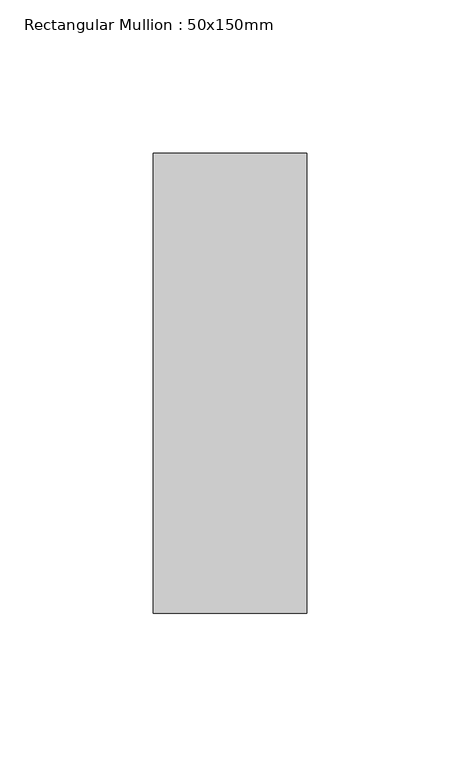
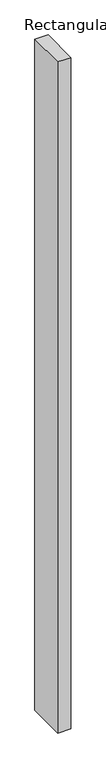
"""IFC4 building model written with IfcOpenShell, lengths in millimetres: member geometry, Rectangular Mullion : 50x150mm."""

from ifc_helpers import new_model, si_unit, frame, origin, place, context, project, spatial, polyline, outline, extrude, source, transform, mapped, element, save


def rectangular_mullion_50x150mm_929c4ac2(model_context):
    return source(origin(), model_context, "Body", "SweptSolid", [
        extrude(outline(polyline([(0.0, 75.0), (0.0, -75.0), (-50.0, -75.0), (-50.0, 75.0), (0.0, 75.0)])), frame((0.0, 0.0, -2700.0), z_axis=(0.0, 0.0, 1.0), x_axis=(1.0, 0.0, 0.0)), (0.0, 0.0, 1.0), 2700.0),
    ])


if __name__ == "__main__":
    model = new_model("IFC4")
    model_context = context("Model", 3, world=origin())
    ifc_project = project(units=[si_unit("LENGTHUNIT", "METRE", prefix="MILLI")], contexts=[model_context])
    site = spatial("IfcSite", under=ifc_project)
    building = spatial("IfcBuilding", under=site)
    placement = place(None, origin())
    rectangular_mullion_50x150mm_shape = rectangular_mullion_50x150mm_929c4ac2(model_context)
    element("IfcMember", 1, ObjectType="Rectangular Mullion : 50x150mm", at=placement, inside=building, context=model_context, shape_type="MappedRepresentation", body=[
        mapped(rectangular_mullion_50x150mm_shape, transform((0.0, 0.0, 0.0), x_axis=(1.0, 0.0, 0.0), y_axis=(0.0, 1.0, 0.0), z_axis=(0.0, 0.0, 1.0))),
    ])
    save(model, "model.ifc")

# Revit data of these elements
# Type "Rectangular Mullion : 50x150mm"
#   Keynote = "H11"
#   built-in parameter 1007304 = 0.492126 (stored number, unit not read)
#   built-in parameter 1007301 = 0.082021 (stored number, unit not read)
#   built-in parameter 1007300 = 0.082021 (stored number, unit not read)
# Element 1 (IfcMember, "Rectangular Mullion : 50x150mm")
#   Materials on its faces: "Aluminium"
# Materials
#   "Aluminium": class "Metal", colour RGB 247 247 247, transparency 0, Description = "Aluminium 6061", Cost = 0
